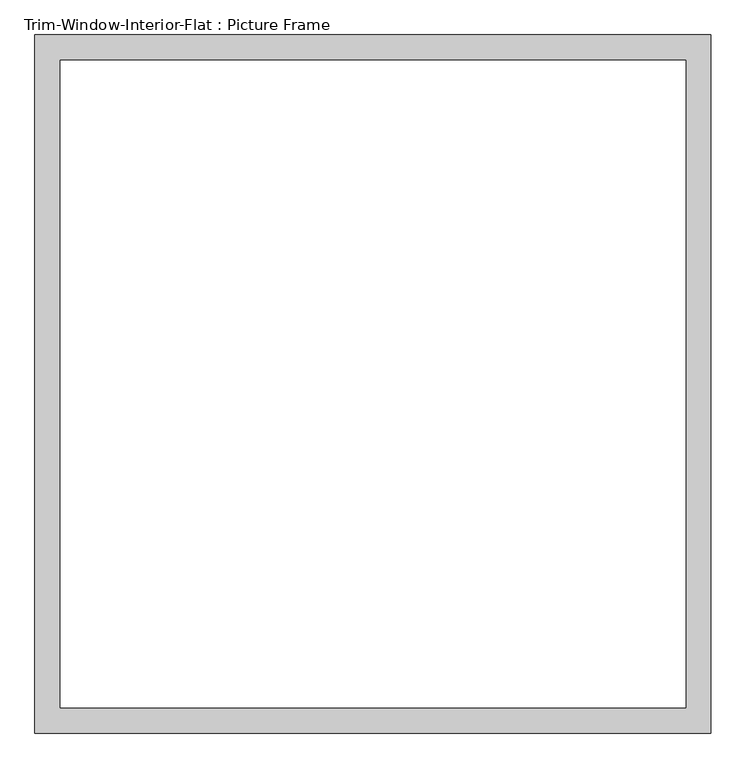
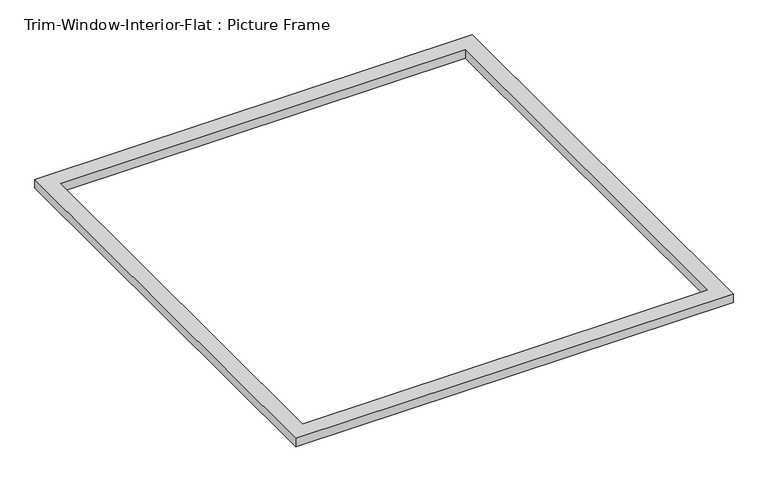
"""IFC4 building model written with IfcOpenShell, lengths in millimetres: proxy geometry, Trim-Window-Interior-Flat : Picture Frame."""

import ifcopenshell
import ifcopenshell.guid

model = None  # the IFC model being written
_history = None  # IfcOwnerHistory: only IFC2X3 demands one
_inside = {}  # id of a spatial element -> (the spatial element, [elements in it])
_under = {}  # id of a project, library or spatial element -> (it, [spatial elements below it])
_declared = {}  # id of a project -> (the project, [libraries it declares])
_typed = {}  # id of a type object -> (the type object, [elements of that type])
_made_of = {}  # id of a material, layer set ... -> (it, [elements and type objects made of it])


def new_model(schema):
    """Start an empty IFC model of exactly this schema.

    Asked for "IFC4X3", IfcOpenShell would pick the latest addendum, in which some entities
    have other attributes; the version numbers below select the first issue.
    IFC2X3 requires an IfcOwnerHistory on every rooted entity: one is made here for all.
    """
    global model, _history
    if schema == "IFC4X3":
        model = ifcopenshell.file(schema_version=(4, 3, 0, 0))
    else:
        model = ifcopenshell.file(schema=schema)
    _inside.clear()
    _under.clear()
    _declared.clear()
    _typed.clear()
    _made_of.clear()
    _history = None
    if model.schema == "IFC2X3":
        org = make("IfcOrganization", Name="unknown")
        user = make(
            "IfcPersonAndOrganization",
            ThePerson=make("IfcPerson", FamilyName="unknown"),
            TheOrganization=org,
        )
        app = make(
            "IfcApplication",
            ApplicationDeveloper=org,
            Version="unknown",
            ApplicationFullName="unknown",
            ApplicationIdentifier="unknown",
        )
        _history = make(
            "IfcOwnerHistory",
            OwningUser=user,
            OwningApplication=app,
            ChangeAction="ADDED",
            CreationDate=0,
        )
    return model


def make(cls, **values):
    """One entity of the class cls with the attributes given. An attribute that is None is left unset."""
    return model.create_entity(
        cls, **{name: value for name, value in values.items() if value is not None}
    )


def rooted(cls, **values):
    """An entity with a GlobalId (a new one), such as an element, a storey or a relation."""
    return make(cls, GlobalId=ifcopenshell.guid.new(), OwnerHistory=_history, **values)


def si_unit(unit_type, name, prefix=None):
    """IfcSIUnit, for example si_unit("LENGTHUNIT", "METRE", prefix="MILLI")."""
    return make("IfcSIUnit", UnitType=unit_type, Prefix=prefix, Name=name)


def assignment(units):
    """IfcUnitAssignment: the units of a project."""
    return None if units is None else make("IfcUnitAssignment", Units=units)


def point(xyz):
    """IfcCartesianPoint."""
    return None if xyz is None else make("IfcCartesianPoint", Coordinates=xyz)


def direction(xyz):
    """IfcDirection."""
    return None if xyz is None else make("IfcDirection", DirectionRatios=xyz)


def frame(location, z_axis=None, x_axis=None):
    """IfcAxis2Placement3D, a coordinate frame: its origin and axes. An axis left out is left unset."""
    return make(
        "IfcAxis2Placement3D",
        Location=point(location),
        Axis=direction(z_axis),
        RefDirection=direction(x_axis),
    )


def origin():
    """The frame at (0, 0, 0) with its axes left unset."""
    return frame((0.0, 0.0, 0.0))


def origin_with_axes():
    """The frame at (0, 0, 0) with the z axis (0, 0, 1) and the x axis (1, 0, 0) written out."""
    return frame((0.0, 0.0, 0.0), z_axis=(0.0, 0.0, 1.0), x_axis=(1.0, 0.0, 0.0))


def place(relative_to, where):
    """IfcLocalPlacement: puts the frame where relative to a parent placement (None: the world)."""
    return make(
        "IfcLocalPlacement", PlacementRelTo=relative_to, RelativePlacement=where
    )


def context(
    kind, dimensions, precision=None, world=None, true_north=None, identifier=None
):
    """IfcGeometricRepresentationContext, for example the 3D "Model" context."""
    return make(
        "IfcGeometricRepresentationContext",
        ContextIdentifier=identifier,
        ContextType=kind,
        CoordinateSpaceDimension=dimensions,
        Precision=precision,
        WorldCoordinateSystem=world,
        TrueNorth=true_north,
    )


def project(units=None, contexts=None):
    """IfcProject with its units and contexts."""
    return rooted(
        "IfcProject",
        Name="project",
        RepresentationContexts=contexts,
        UnitsInContext=assignment(units),
    )


def spatial(cls, under=None, at=None, **own):
    """A site, building, storey or space (cls), placed at a placement, below another one or the project."""
    s = rooted(cls, ObjectPlacement=at, **own)
    if under is not None:
        _under.setdefault(under.id(), (under, []))[1].append(s)
    return s


def polyline(points):
    """IfcPolyline through the points."""
    return make("IfcPolyline", Points=[point(p) for p in points])


def outline(outer, holes=None, kind="AREA"):
    """IfcArbitraryClosedProfileDef: a profile drawn as a closed curve; with holes, ...WithVoids."""
    if holes is None:
        return make("IfcArbitraryClosedProfileDef", ProfileType=kind, OuterCurve=outer)
    return make(
        "IfcArbitraryProfileDefWithVoids",
        ProfileType=kind,
        OuterCurve=outer,
        InnerCurves=holes,
    )


def extrude(swept, where, along, depth):
    """IfcExtrudedAreaSolid: the profile swept, set in the frame where, extruded along a direction by depth."""
    return make(
        "IfcExtrudedAreaSolid",
        SweptArea=swept,
        Position=where,
        ExtrudedDirection=direction(along),
        Depth=depth,
    )


def shape(context_of_items, identifier, shape_type, items):
    """IfcShapeRepresentation: the items that make up one representation, for example the "Body"."""
    return make(
        "IfcShapeRepresentation",
        ContextOfItems=context_of_items,
        RepresentationIdentifier=identifier,
        RepresentationType=shape_type,
        Items=items,
    )


def source(mapping_origin, context_of_items, identifier, shape_type, items):
    """IfcRepresentationMap: a shape defined once, which mapped items show again and again."""
    return make(
        "IfcRepresentationMap",
        MappingOrigin=mapping_origin,
        MappedRepresentation=shape(context_of_items, identifier, shape_type, items),
    )


def transform(
    local_origin,
    x_axis=None,
    y_axis=None,
    z_axis=None,
    scale=None,
    scale2=None,
    scale3=None,
    uniform=True,
):
    """IfcCartesianTransformationOperator3D, or its non-uniform kind. x_axis, y_axis, z_axis: its Axis1, 2, 3."""
    if uniform:
        return make(
            "IfcCartesianTransformationOperator3D",
            Axis1=direction(x_axis),
            Axis2=direction(y_axis),
            LocalOrigin=point(local_origin),
            Scale=scale,
            Axis3=direction(z_axis),
        )
    return make(
        "IfcCartesianTransformationOperator3DnonUniform",
        Axis1=direction(x_axis),
        Axis2=direction(y_axis),
        LocalOrigin=point(local_origin),
        Scale=scale,
        Axis3=direction(z_axis),
        Scale2=scale2,
        Scale3=scale3,
    )


def mapped(mapping_source, mapping_target):
    """IfcMappedItem: shows the shape of a source again, moved by a transform."""
    return make(
        "IfcMappedItem", MappingSource=mapping_source, MappingTarget=mapping_target
    )


def made_of(thing, what):
    """Note that an element or type object is made of a material, layer set ...; save() writes the relation."""
    if what is not None:
        _made_of.setdefault(what.id(), (what, []))[1].append(thing)
    return thing


def element(
    cls,
    number,
    at=None,
    inside=None,
    cuts=None,
    type_object=None,
    material=None,
    context=None,
    identifier="Body",
    shape_type=None,
    held_by="IfcProductDefinitionShape",
    body=None,
    shapes=None,
    **own,
):
    """One element of the class cls, such as IfcWall. Its Tag is "e" and its number.

    at: its placement. inside: the storey or other place that contains it. cuts: it is an
    opening in that element (IfcRelVoidsElement). A single representation is given by context,
    identifier, shape_type and body (its items); several are given by shapes. held_by: the class
    of the entity that holds the representations. save() writes the other relations.
    """
    e = rooted(cls, Tag="e%d" % number, ObjectPlacement=at, **own)
    if body is not None:
        shapes = [shape(context, identifier, shape_type, body)]
    if shapes is not None:
        e.Representation = make(held_by, Representations=shapes)
    if inside is not None:
        _inside.setdefault(inside.id(), (inside, []))[1].append(e)
    if cuts is not None:
        rooted(
            "IfcRelVoidsElement", RelatingBuildingElement=cuts, RelatedOpeningElement=e
        )
    if type_object is not None:
        _typed.setdefault(type_object.id(), (type_object, []))[1].append(e)
    return made_of(e, material)


def aggregate(whole, parts):
    """IfcRelAggregates: a whole, such as a stair, and the parts it consists of."""
    return rooted("IfcRelAggregates", RelatingObject=whole, RelatedObjects=parts)


def save(model, path):
    """Write the relations noted so far, then the file.

    IfcRelAggregates (storeys below a building ...), IfcRelContainedInSpatialStructure (elements
    in a storey), IfcRelDefinesByType, IfcRelAssociatesMaterial and IfcRelDeclares: one each for
    every whole, place, type object, material and project.
    """
    for whole, parts in _under.values():
        aggregate(whole, parts)
    for where, things in _inside.values():
        rooted(
            "IfcRelContainedInSpatialStructure",
            RelatedElements=things,
            RelatingStructure=where,
        )
    for kind, things in _typed.values():
        rooted("IfcRelDefinesByType", RelatedObjects=things, RelatingType=kind)
    for what, things in _made_of.values():
        rooted("IfcRelAssociatesMaterial", RelatedObjects=things, RelatingMaterial=what)
    for by, libraries in _declared.values():
        rooted("IfcRelDeclares", RelatingContext=by, RelatedDefinitions=libraries)
    model.write(path)


def trim_window_interior_flat_picture_frame_c6096a02(model_context):
    return source(origin(), model_context, "Body", "SweptSolid", [
        extrude(outline(polyline([(768.35, 44.45), (768.35, -1543.05), (-768.35, -1543.05), (-768.35, 44.45), (768.35, 44.45)]), holes=[polyline([(711.2, -12.7), (-711.2, -12.7), (-711.2, -1485.9), (711.2, -1485.9), (711.2, -12.7)])]), origin_with_axes(), (0.0, 0.0, 1.0), 31.75),
    ])


if __name__ == "__main__":
    model = new_model("IFC4")
    model_context = context("Model", 3, world=origin())
    ifc_project = project(units=[si_unit("LENGTHUNIT", "METRE", prefix="MILLI")], contexts=[model_context])
    site = spatial("IfcSite", under=ifc_project)
    building = spatial("IfcBuilding", under=site)
    placement = place(None, origin())
    trim_window_interior_flat_picture_frame_shape = trim_window_interior_flat_picture_frame_c6096a02(model_context)
    element("IfcBuildingElementProxy", 1, Name="Trim-Window-Interior-Flat : Picture Frame", ObjectType="Trim-Window-Interior-Flat : Picture Frame", at=placement, inside=building, context=model_context, shape_type="MappedRepresentation", body=[
        mapped(trim_window_interior_flat_picture_frame_shape, transform((0.0, 0.0, 0.0), x_axis=(1.0, 0.0, 0.0), y_axis=(0.0, 1.0, 0.0), z_axis=(0.0, 0.0, 1.0))),
    ])
    save(model, "model.ifc")

# Revit data of these elements
# Type "Trim-Window-Interior-Flat : Picture Frame"
#   Trim Thickness_Picture Frame = 0' - 1 1/4"
#   Trim Width = 0' - 2 1/4"
#   Trim Thickness_with Sill = 0' - 0 3/4"
#   Sill Thickness = 0' - 1 1/4"
#   Opening Width [instance default] = 2' - 0"
#   Opening Height [instance default] = 3' - 0"
#   Default Elevation = 4' - 0"
#   Sill = no
#   Picture Frame = yes
#   Trim Material [instance default] = none
# Element 1 (IfcBuildingElementProxy, "Trim-Window-Interior-Flat : Picture Frame")
#   Opening Width = 4' - 9"
#   Opening Height = 4' - 11"
#   Trim Material = Wood - Stained
#   Materials on its faces: "Wood - Stained"
# Materials
#   "Wood - Stained": class "Wood", colour RGB 224 178 126, transparency 0, Cost = 0
